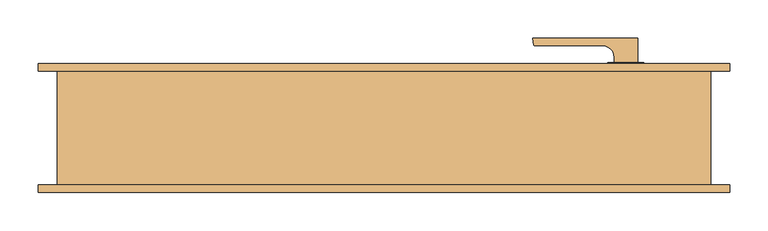
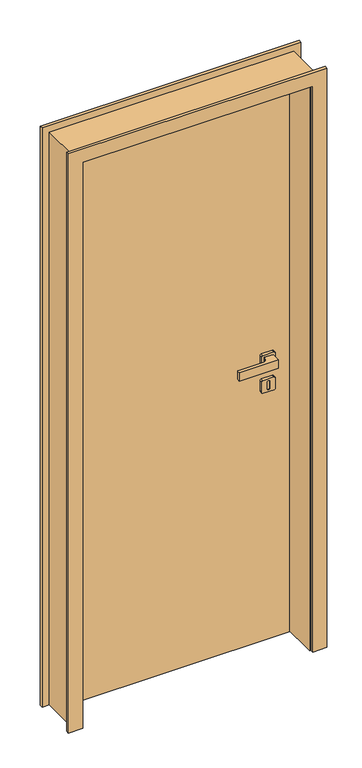
"""IFC4 building model written with IfcOpenShell, lengths in millimetres: door geometry, porta multiplas_growarq : porta giro simples 80 cm_growarq."""

import ifcopenshell
import ifcopenshell.guid

model = None  # the IFC model being written
_history = None  # IfcOwnerHistory: only IFC2X3 demands one
_inside = {}  # id of a spatial element -> (the spatial element, [elements in it])
_under = {}  # id of a project, library or spatial element -> (it, [spatial elements below it])
_declared = {}  # id of a project -> (the project, [libraries it declares])
_typed = {}  # id of a type object -> (the type object, [elements of that type])
_made_of = {}  # id of a material, layer set ... -> (it, [elements and type objects made of it])


def new_model(schema):
    """Start an empty IFC model of exactly this schema.

    Asked for "IFC4X3", IfcOpenShell would pick the latest addendum, in which some entities
    have other attributes; the version numbers below select the first issue.
    IFC2X3 requires an IfcOwnerHistory on every rooted entity: one is made here for all.
    """
    global model, _history
    if schema == "IFC4X3":
        model = ifcopenshell.file(schema_version=(4, 3, 0, 0))
    else:
        model = ifcopenshell.file(schema=schema)
    _inside.clear()
    _under.clear()
    _declared.clear()
    _typed.clear()
    _made_of.clear()
    _history = None
    if model.schema == "IFC2X3":
        org = make("IfcOrganization", Name="unknown")
        user = make(
            "IfcPersonAndOrganization",
            ThePerson=make("IfcPerson", FamilyName="unknown"),
            TheOrganization=org,
        )
        app = make(
            "IfcApplication",
            ApplicationDeveloper=org,
            Version="unknown",
            ApplicationFullName="unknown",
            ApplicationIdentifier="unknown",
        )
        _history = make(
            "IfcOwnerHistory",
            OwningUser=user,
            OwningApplication=app,
            ChangeAction="ADDED",
            CreationDate=0,
        )
    return model


def make(cls, **values):
    """One entity of the class cls with the attributes given. An attribute that is None is left unset."""
    return model.create_entity(
        cls, **{name: value for name, value in values.items() if value is not None}
    )


def rooted(cls, **values):
    """An entity with a GlobalId (a new one), such as an element, a storey or a relation."""
    return make(cls, GlobalId=ifcopenshell.guid.new(), OwnerHistory=_history, **values)


def si_unit(unit_type, name, prefix=None):
    """IfcSIUnit, for example si_unit("LENGTHUNIT", "METRE", prefix="MILLI")."""
    return make("IfcSIUnit", UnitType=unit_type, Prefix=prefix, Name=name)


def assignment(units):
    """IfcUnitAssignment: the units of a project."""
    return None if units is None else make("IfcUnitAssignment", Units=units)


def point(xyz):
    """IfcCartesianPoint."""
    return None if xyz is None else make("IfcCartesianPoint", Coordinates=xyz)


def direction(xyz):
    """IfcDirection."""
    return None if xyz is None else make("IfcDirection", DirectionRatios=xyz)


def frame(location, z_axis=None, x_axis=None):
    """IfcAxis2Placement3D, a coordinate frame: its origin and axes. An axis left out is left unset."""
    return make(
        "IfcAxis2Placement3D",
        Location=point(location),
        Axis=direction(z_axis),
        RefDirection=direction(x_axis),
    )


def frame_2d(location, x_axis=None):
    """IfcAxis2Placement2D, a coordinate frame in the plane: its origin and x axis."""
    return make(
        "IfcAxis2Placement2D", Location=point(location), RefDirection=direction(x_axis)
    )


def origin():
    """The frame at (0, 0, 0) with its axes left unset."""
    return frame((0.0, 0.0, 0.0))


def origin_with_axes():
    """The frame at (0, 0, 0) with the z axis (0, 0, 1) and the x axis (1, 0, 0) written out."""
    return frame((0.0, 0.0, 0.0), z_axis=(0.0, 0.0, 1.0), x_axis=(1.0, 0.0, 0.0))


def place(relative_to, where):
    """IfcLocalPlacement: puts the frame where relative to a parent placement (None: the world)."""
    return make(
        "IfcLocalPlacement", PlacementRelTo=relative_to, RelativePlacement=where
    )


def context(
    kind, dimensions, precision=None, world=None, true_north=None, identifier=None
):
    """IfcGeometricRepresentationContext, for example the 3D "Model" context."""
    return make(
        "IfcGeometricRepresentationContext",
        ContextIdentifier=identifier,
        ContextType=kind,
        CoordinateSpaceDimension=dimensions,
        Precision=precision,
        WorldCoordinateSystem=world,
        TrueNorth=true_north,
    )


def project(units=None, contexts=None):
    """IfcProject with its units and contexts."""
    return rooted(
        "IfcProject",
        Name="project",
        RepresentationContexts=contexts,
        UnitsInContext=assignment(units),
    )


def spatial(cls, under=None, at=None, **own):
    """A site, building, storey or space (cls), placed at a placement, below another one or the project."""
    s = rooted(cls, ObjectPlacement=at, **own)
    if under is not None:
        _under.setdefault(under.id(), (under, []))[1].append(s)
    return s


def polyline(points):
    """IfcPolyline through the points."""
    return make("IfcPolyline", Points=[point(p) for p in points])


def circle_curve(where, radius):
    """IfcCircle in the frame where."""
    return make("IfcCircle", Position=where, Radius=radius)


def trimmed(basis, trim1, trim2, sense, master):
    """IfcTrimmedCurve: the piece of a basis curve between two trims."""
    return make(
        "IfcTrimmedCurve",
        BasisCurve=basis,
        Trim1=trim1,
        Trim2=trim2,
        SenseAgreement=sense,
        MasterRepresentation=master,
    )


def segment(curve, same_sense, transition):
    """IfcCompositeCurveSegment."""
    return make(
        "IfcCompositeCurveSegment",
        Transition=transition,
        SameSense=same_sense,
        ParentCurve=curve,
    )


def composite_curve(segments, self_intersect=None):
    """IfcCompositeCurve: segments joined end to end."""
    return make("IfcCompositeCurve", Segments=segments, SelfIntersect=self_intersect)


def outline(outer, holes=None, kind="AREA"):
    """IfcArbitraryClosedProfileDef: a profile drawn as a closed curve; with holes, ...WithVoids."""
    if holes is None:
        return make("IfcArbitraryClosedProfileDef", ProfileType=kind, OuterCurve=outer)
    return make(
        "IfcArbitraryProfileDefWithVoids",
        ProfileType=kind,
        OuterCurve=outer,
        InnerCurves=holes,
    )


def extrude(swept, where, along, depth):
    """IfcExtrudedAreaSolid: the profile swept, set in the frame where, extruded along a direction by depth."""
    return make(
        "IfcExtrudedAreaSolid",
        SweptArea=swept,
        Position=where,
        ExtrudedDirection=direction(along),
        Depth=depth,
    )


def shape(context_of_items, identifier, shape_type, items):
    """IfcShapeRepresentation: the items that make up one representation, for example the "Body"."""
    return make(
        "IfcShapeRepresentation",
        ContextOfItems=context_of_items,
        RepresentationIdentifier=identifier,
        RepresentationType=shape_type,
        Items=items,
    )


def source(mapping_origin, context_of_items, identifier, shape_type, items):
    """IfcRepresentationMap: a shape defined once, which mapped items show again and again."""
    return make(
        "IfcRepresentationMap",
        MappingOrigin=mapping_origin,
        MappedRepresentation=shape(context_of_items, identifier, shape_type, items),
    )


def transform(
    local_origin,
    x_axis=None,
    y_axis=None,
    z_axis=None,
    scale=None,
    scale2=None,
    scale3=None,
    uniform=True,
):
    """IfcCartesianTransformationOperator3D, or its non-uniform kind. x_axis, y_axis, z_axis: its Axis1, 2, 3."""
    if uniform:
        return make(
            "IfcCartesianTransformationOperator3D",
            Axis1=direction(x_axis),
            Axis2=direction(y_axis),
            LocalOrigin=point(local_origin),
            Scale=scale,
            Axis3=direction(z_axis),
        )
    return make(
        "IfcCartesianTransformationOperator3DnonUniform",
        Axis1=direction(x_axis),
        Axis2=direction(y_axis),
        LocalOrigin=point(local_origin),
        Scale=scale,
        Axis3=direction(z_axis),
        Scale2=scale2,
        Scale3=scale3,
    )


def mapped(mapping_source, mapping_target):
    """IfcMappedItem: shows the shape of a source again, moved by a transform."""
    return make(
        "IfcMappedItem", MappingSource=mapping_source, MappingTarget=mapping_target
    )


def made_of(thing, what):
    """Note that an element or type object is made of a material, layer set ...; save() writes the relation."""
    if what is not None:
        _made_of.setdefault(what.id(), (what, []))[1].append(thing)
    return thing


def element(
    cls,
    number,
    at=None,
    inside=None,
    cuts=None,
    type_object=None,
    material=None,
    context=None,
    identifier="Body",
    shape_type=None,
    held_by="IfcProductDefinitionShape",
    body=None,
    shapes=None,
    **own,
):
    """One element of the class cls, such as IfcWall. Its Tag is "e" and its number.

    at: its placement. inside: the storey or other place that contains it. cuts: it is an
    opening in that element (IfcRelVoidsElement). A single representation is given by context,
    identifier, shape_type and body (its items); several are given by shapes. held_by: the class
    of the entity that holds the representations. save() writes the other relations.
    """
    e = rooted(cls, Tag="e%d" % number, ObjectPlacement=at, **own)
    if body is not None:
        shapes = [shape(context, identifier, shape_type, body)]
    if shapes is not None:
        e.Representation = make(held_by, Representations=shapes)
    if inside is not None:
        _inside.setdefault(inside.id(), (inside, []))[1].append(e)
    if cuts is not None:
        rooted(
            "IfcRelVoidsElement", RelatingBuildingElement=cuts, RelatedOpeningElement=e
        )
    if type_object is not None:
        _typed.setdefault(type_object.id(), (type_object, []))[1].append(e)
    return made_of(e, material)


def aggregate(whole, parts):
    """IfcRelAggregates: a whole, such as a stair, and the parts it consists of."""
    return rooted("IfcRelAggregates", RelatingObject=whole, RelatedObjects=parts)


def save(model, path):
    """Write the relations noted so far, then the file.

    IfcRelAggregates (storeys below a building ...), IfcRelContainedInSpatialStructure (elements
    in a storey), IfcRelDefinesByType, IfcRelAssociatesMaterial and IfcRelDeclares: one each for
    every whole, place, type object, material and project.
    """
    for whole, parts in _under.values():
        aggregate(whole, parts)
    for where, things in _inside.values():
        rooted(
            "IfcRelContainedInSpatialStructure",
            RelatedElements=things,
            RelatingStructure=where,
        )
    for kind, things in _typed.values():
        rooted("IfcRelDefinesByType", RelatedObjects=things, RelatingType=kind)
    for what, things in _made_of.values():
        rooted("IfcRelAssociatesMaterial", RelatedObjects=things, RelatingMaterial=what)
    for by, libraries in _declared.values():
        rooted("IfcRelDeclares", RelatingContext=by, RelatedDefinitions=libraries)
    model.write(path)


def plane_surface(at):
    """IfcPlane: the flat surface through the origin of the frame at, square to its z axis."""
    return make("IfcPlane", Position=at)


def cylinder_surface(at, radius):
    """IfcCylindricalSurface: all points at the distance radius from the z axis of the frame at."""
    return make("IfcCylindricalSurface", Position=at, Radius=radius)


def revolved_surface(curve, axis_point, axis_direction):
    """IfcSurfaceOfRevolution: the curve turned about the line through axis_point along axis_direction."""
    return make(
        "IfcSurfaceOfRevolution",
        SweptCurve=make("IfcArbitraryOpenProfileDef", ProfileType="CURVE", Curve=curve),
        AxisPosition=make("IfcAxis1Placement", Location=point(axis_point), Axis=direction(axis_direction)),
    )


def advanced_brep(points, edges, surfaces, faces):
    """IfcAdvancedBrep: a solid bounded by faces that lie on surfaces and meet in shared edges.

    An edge is (start, end): straight between two places in points (the first is 0);
    or (start, end, curve); or (start, end, curve, False) where it runs against its curve.
    A face is (place in surfaces, loops), or (place, loops, False) where it looks against
    its surface's normal. A loop lists edges by number (the first is 1), with a minus sign
    where the edge is run from its end to its start. The first loop is the outer one.
    """
    corners = [point(p) for p in points]
    vertices = [make("IfcVertexPoint", VertexGeometry=c) for c in corners]
    made = []
    for start, end, *more in edges:
        made.append(
            make(
                "IfcEdgeCurve",
                EdgeStart=vertices[start],
                EdgeEnd=vertices[end],
                EdgeGeometry=more[0] if more else make("IfcPolyline", Points=[corners[start], corners[end]]),
                SameSense=more[1] if len(more) > 1 else True,
            )
        )
    hull = []
    for where, loops, *sense in faces:
        bounds = []
        for j, loop in enumerate(loops):
            ring = [make("IfcOrientedEdge", EdgeElement=made[abs(k) - 1], Orientation=k > 0) for k in loop]
            bounds.append(
                make(
                    "IfcFaceOuterBound" if j == 0 else "IfcFaceBound",
                    Bound=make("IfcEdgeLoop", EdgeList=ring),
                    Orientation=True,
                )
            )
        hull.append(make("IfcAdvancedFace", Bounds=bounds, FaceSurface=surfaces[where], SameSense=sense[0] if sense else True))
    return make("IfcAdvancedBrep", Outer=make("IfcClosedShell", CfsFaces=hull))


def door_262d71ed(model_context):
    return source(origin(), model_context, "Body", "SolidModel", [
        advanced_brep(
        [(337.5247906, 86.0, 975.2140175), (341.5247906, 86.0, 971.2140175), (341.5247906, 86.0, 932.3348635), (337.5247906, 86.0, 928.3348635), (298.475196, 86.0, 928.3348635), (294.475196, 86.0, 932.3348635), (294.475196, 86.0, 971.2071442), (298.4820692, 86.0, 975.2140175), (323.0036235, 86.0, 963.1453546), (312.9935514, 86.0, 963.1453546), (312.9935514, 86.0, 940.4035264), (323.0036235, 86.0, 940.4035264), (337.5247906, 75.0, 975.2140175), (298.4820692, 75.0, 975.2140175), (294.475196, 75.0, 971.2071442), (294.475196, 75.0, 932.3348635), (298.475196, 75.0, 928.3348635), (337.5247906, 75.0, 928.3348635), (341.5247906, 75.0, 932.3348635), (341.5247906, 75.0, 971.2140175), (323.0036235, 84.0, 940.4035264), (312.9935514, 84.0, 940.4035264), (312.9935514, 84.0, 963.1453546), (323.0036235, 84.0, 963.1453546)],
        [
            (0, 1, circle_curve(frame((337.5247906, 86.0, 971.2140175), z_axis=(0.0, 1.0, 0.0), x_axis=(1.0, 0.0, 0.0)), 4.0)),
            (1, 2),
            (2, 3, circle_curve(frame((337.5247906, 86.0, 932.3348635), z_axis=(0.0, 1.0, 0.0), x_axis=(1.0, 0.0, 0.0)), 4.0)),
            (3, 4),
            (4, 5, circle_curve(frame((298.475196, 86.0, 932.3348635), z_axis=(0.0, 1.0, 0.0), x_axis=(1.0, 0.0, 0.0)), 4.0)),
            (5, 6),
            (6, 7, circle_curve(frame((298.4820692, 86.0, 971.2071442), z_axis=(0.0, 1.0, 0.0), x_axis=(1.0, 0.0, 0.0)), 4.0068732)),
            (7, 0),
            (8, 9, circle_curve(frame((317.9985874, 86.0, 963.1453546), z_axis=(0.0, -1.0, 0.0), x_axis=(1.0, 0.0, 0.0)), 5.0050361)),
            (9, 10),
            (10, 11, circle_curve(frame((317.9985874, 86.0, 940.4035264), z_axis=(0.0, -1.0, 0.0), x_axis=(1.0, 0.0, 0.0)), 5.0050361)),
            (11, 8),
            (12, 13),
            (13, 14, circle_curve(frame((298.4820692, 75.0, 971.2071442), z_axis=(0.0, -1.0, 0.0), x_axis=(1.0, 0.0, 0.0)), 4.0068732)),
            (14, 15),
            (15, 16, circle_curve(frame((298.475196, 75.0, 932.3348635), z_axis=(0.0, -1.0, 0.0), x_axis=(1.0, 0.0, 0.0)), 4.0)),
            (16, 17),
            (17, 18, circle_curve(frame((337.5247906, 75.0, 932.3348635), z_axis=(0.0, -1.0, 0.0), x_axis=(1.0, 0.0, 0.0)), 4.0)),
            (18, 19),
            (19, 12, circle_curve(frame((337.5247906, 75.0, 971.2140175), z_axis=(0.0, -1.0, 0.0), x_axis=(1.0, 0.0, 0.0)), 4.0)),
            (7, 13),
            (12, 0),
            (6, 14),
            (5, 15),
            (4, 16),
            (3, 17),
            (2, 18),
            (1, 19),
            (20, 21, circle_curve(frame((317.9985874, 84.0, 940.4035264), z_axis=(0.0, 1.0, 0.0), x_axis=(1.0, 0.0, 0.0)), 5.0050361)),
            (21, 22),
            (22, 23, circle_curve(frame((317.9985874, 84.0, 963.1453546), z_axis=(0.0, 1.0, 0.0), x_axis=(1.0, 0.0, 0.0)), 5.0050361)),
            (23, 20),
            (23, 8),
            (11, 20),
            (21, 10),
            (9, 22),
        ],
        [
            plane_surface(frame((298.4781039, 86.0, 975.2140175), z_axis=(0.0, 1.0, 0.0), x_axis=(-1.0, 0.0, 0.0))),
            plane_surface(frame((298.4781039, 75.0, 975.2140175), z_axis=(0.0, -1.0, 0.0), x_axis=(1.0, 0.0, 0.0))),
            plane_surface(frame((337.5247906, 86.0, 975.2140175), z_axis=(0.0, 0.0, 1.0), x_axis=(0.0, -1.0, 0.0))),
            cylinder_surface(frame((298.4820692, 75.0, 971.2071442), z_axis=(0.0, 1.0, 0.0), x_axis=(1.0, 0.0, 0.0)), 4.0068732),
            plane_surface(frame((294.475196, 86.0, 971.2071442), z_axis=(-1.0, 0.0, 0.0), x_axis=(0.0, -1.0, 0.0))),
            cylinder_surface(frame((298.475196, 75.0, 932.3348635), z_axis=(0.0, 1.0, 0.0), x_axis=(1.0, 0.0, 0.0)), 4.0),
            plane_surface(frame((298.475196, 86.0, 928.3348635), z_axis=(0.0, 0.0, -1.0), x_axis=(0.0, -1.0, 0.0))),
            cylinder_surface(frame((337.5247906, 75.0, 932.3348635), z_axis=(0.0, 1.0, 0.0), x_axis=(1.0, 0.0, 0.0)), 4.0),
            plane_surface(frame((341.5247906, 86.0, 932.3348635), z_axis=(1.0, 0.0, 0.0), x_axis=(0.0, -1.0, 0.0))),
            cylinder_surface(frame((337.5247906, 75.0, 971.2140175), z_axis=(0.0, 1.0, 0.0), x_axis=(1.0, 0.0, 0.0)), 4.0),
            plane_surface(frame((323.0036235, 84.0, 952.9958878), z_axis=(0.0, 1.0, 0.0), x_axis=(0.0, 0.0, -1.0))),
            plane_surface(frame((323.0036235, 86.0, 940.4035264), z_axis=(-1.0, 0.0, 0.0), x_axis=(0.0, -1.0, 0.0))),
            plane_surface(frame((312.9935514, 86.0, 963.1453546), z_axis=(1.0, 0.0, 0.0), x_axis=(0.0, -1.0, 0.0))),
            revolved_surface(polyline([(323.0036235, 86.0, 940.4035264), (323.0036235, 84.0, 940.4035264)]), (317.9985874, 84.0, 940.4035264), (0.0, 1.0, 0.0)),
            revolved_surface(polyline([(323.0036235, 86.0, 963.1453546), (323.0036235, 84.0, 963.1453546)]), (317.9985874, 84.0, 963.1453546), (0.0, 1.0, 0.0)),
        ],
        [
            (0, [[1, 2, 3, 4, 5, 6, 7, 8], [9, 10, 11, 12]]),
            (1, [[13, 14, 15, 16, 17, 18, 19, 20]]),
            (2, [[21, -13, 22, -8]]),
            (3, [[23, -14, -21, -7]]),
            (4, [[24, -15, -23, -6]]),
            (5, [[25, -16, -24, -5]]),
            (6, [[26, -17, -25, -4]]),
            (7, [[27, -18, -26, -3]]),
            (8, [[28, -19, -27, -2]]),
            (9, [[-22, -20, -28, -1]]),
            (10, [[29, 30, 31, 32]]),
            (11, [[33, -12, 34, -32]]),
            (12, [[35, -10, 36, -30]]),
            (13, [[-34, -11, -35, -29]]),
            (14, [[-36, -9, -33, -31]]),
        ],
    ),
        advanced_brep(
        [(337.5247906, 86.0, 1068.227973), (341.5247906, 86.0, 1064.227973), (341.5247906, 86.0, 1025.3488191), (337.5247906, 86.0, 1021.3488191), (298.475196, 86.0, 1021.3488191), (294.475196, 86.0, 1025.3488191), (294.475196, 86.0, 1064.2210998), (298.4820692, 86.0, 1068.227973), (337.5247906, 75.0, 1068.227973), (298.4820692, 75.0, 1068.227973), (294.475196, 75.0, 1064.2210998), (294.475196, 75.0, 1025.3488191), (298.475196, 75.0, 1021.3488191), (337.5247906, 75.0, 1021.3488191), (341.5247906, 75.0, 1025.3488191), (341.5247906, 75.0, 1064.227973)],
        [
            (0, 1, circle_curve(frame((337.5247906, 86.0, 1064.227973), z_axis=(0.0, 1.0, 0.0), x_axis=(1.0, 0.0, 0.0)), 4.0)),
            (1, 2),
            (2, 3, circle_curve(frame((337.5247906, 86.0, 1025.3488191), z_axis=(0.0, 1.0, 0.0), x_axis=(1.0, 0.0, 0.0)), 4.0)),
            (3, 4),
            (4, 5, circle_curve(frame((298.475196, 86.0, 1025.3488191), z_axis=(0.0, 1.0, 0.0), x_axis=(1.0, 0.0, 0.0)), 4.0)),
            (5, 6),
            (6, 7, circle_curve(frame((298.4820692, 86.0, 1064.2210998), z_axis=(0.0, 1.0, 0.0), x_axis=(1.0, 0.0, 0.0)), 4.0068732)),
            (7, 0),
            (8, 9),
            (9, 10, circle_curve(frame((298.4820692, 75.0, 1064.2210998), z_axis=(0.0, -1.0, 0.0), x_axis=(1.0, 0.0, 0.0)), 4.0068732)),
            (10, 11),
            (11, 12, circle_curve(frame((298.475196, 75.0, 1025.3488191), z_axis=(0.0, -1.0, 0.0), x_axis=(1.0, 0.0, 0.0)), 4.0)),
            (12, 13),
            (13, 14, circle_curve(frame((337.5247906, 75.0, 1025.3488191), z_axis=(0.0, -1.0, 0.0), x_axis=(1.0, 0.0, 0.0)), 4.0)),
            (14, 15),
            (15, 8, circle_curve(frame((337.5247906, 75.0, 1064.227973), z_axis=(0.0, -1.0, 0.0), x_axis=(1.0, 0.0, 0.0)), 4.0)),
            (7, 9),
            (8, 0),
            (6, 10),
            (5, 11),
            (4, 12),
            (3, 13),
            (2, 14),
            (1, 15),
        ],
        [
            plane_surface(frame((298.4781039, 86.0, 975.2140175), z_axis=(0.0, 1.0, 0.0), x_axis=(-1.0, 0.0, 0.0))),
            plane_surface(frame((298.4781039, 75.0, 975.2140175), z_axis=(0.0, -1.0, 0.0), x_axis=(1.0, 0.0, 0.0))),
            plane_surface(frame((337.5247906, 86.0, 1068.227973), z_axis=(0.0, 0.0, 1.0), x_axis=(0.0, -1.0, 0.0))),
            cylinder_surface(frame((298.4820692, 75.0, 1064.2210998), z_axis=(0.0, 1.0, 0.0), x_axis=(1.0, 0.0, 0.0)), 4.0068732),
            plane_surface(frame((294.475196, 86.0, 1064.2210998), z_axis=(-1.0, 0.0, 0.0), x_axis=(0.0, -1.0, 0.0))),
            cylinder_surface(frame((298.475196, 75.0, 1025.3488191), z_axis=(0.0, 1.0, 0.0), x_axis=(1.0, 0.0, 0.0)), 4.0),
            plane_surface(frame((298.475196, 86.0, 1021.3488191), z_axis=(0.0, 0.0, -1.0), x_axis=(0.0, -1.0, 0.0))),
            cylinder_surface(frame((337.5247906, 75.0, 1025.3488191), z_axis=(0.0, 1.0, 0.0), x_axis=(1.0, 0.0, 0.0)), 4.0),
            plane_surface(frame((341.5247906, 86.0, 1025.3488191), z_axis=(1.0, 0.0, 0.0), x_axis=(0.0, -1.0, 0.0))),
            cylinder_surface(frame((337.5247906, 75.0, 1064.227973), z_axis=(0.0, 1.0, 0.0), x_axis=(1.0, 0.0, 0.0)), 4.0),
        ],
        [
            (0, [[1, 2, 3, 4, 5, 6, 7, 8]]),
            (1, [[9, 10, 11, 12, 13, 14, 15, 16]]),
            (2, [[17, -9, 18, -8]]),
            (3, [[19, -10, -17, -7]]),
            (4, [[20, -11, -19, -6]]),
            (5, [[21, -12, -20, -5]]),
            (6, [[22, -13, -21, -4]]),
            (7, [[23, -14, -22, -3]]),
            (8, [[24, -15, -23, -2]]),
            (9, [[-18, -16, -24, -1]]),
        ],
    ),
        extrude(outline(composite_curve([segment(polyline([(333.5247906, 118.5150355), (333.5247906, 86.7793682), (302.475196, 86.7793682), (302.475196, 93.5981558)]), True, "CONTINUOUS"), segment(trimmed(circle_curve(frame_2d((287.4483579, 93.5981558)), 15.0268381), [point((302.475196, 93.5981558))], [point((287.4483579, 108.6249939))], True, "CARTESIAN"), True, "CONTINUOUS"), segment(polyline([(287.4483579, 108.6249939), (198.1590205, 108.6249939)]), True, "CONTINUOUS"), segment(trimmed(circle_curve(frame_2d((198.1590205, 109.6372538)), 1.0122598), [point((198.1590205, 108.6249939))], [point((197.1621392, 109.4614767))], False, "CARTESIAN"), True, "CONTINUOUS"), segment(polyline([(197.1621392, 109.4614767), (195.5657525, 118.5150355), (333.5247906, 118.5150355)]), True, "CONTINUOUS")], self_intersect=False)), frame((0.0, 0.0, 1029.3488191), z_axis=(0.0, 0.0, 1.0), x_axis=(1.0, 0.0, 0.0)), (0.0, 0.0, 1.0), 30.8791539),
        advanced_brep(
        [(337.5247906, 34.0, 975.2140175), (298.4820692, 34.0, 975.2140175), (294.475196, 34.0, 971.2071442), (294.475196, 34.0, 932.3348635), (298.475196, 34.0, 928.3348635), (337.5247906, 34.0, 928.3348635), (341.5247906, 34.0, 932.3348635), (341.5247906, 34.0, 971.2140175), (323.0036235, 34.0, 963.1453546), (323.0036235, 34.0, 940.4035264), (312.9935514, 34.0, 940.4035264), (312.9935514, 34.0, 963.1453546), (337.5247906, 45.0, 975.2140175), (341.5247906, 45.0, 971.2140175), (341.5247906, 45.0, 932.3348635), (337.5247906, 45.0, 928.3348635), (298.475196, 45.0, 928.3348635), (294.475196, 45.0, 932.3348635), (294.475196, 45.0, 971.2071442), (298.4820692, 45.0, 975.2140175), (323.0036235, 36.0, 940.4035264), (323.0036235, 36.0, 963.1453546), (312.9935514, 36.0, 963.1453546), (312.9935514, 36.0, 940.4035264)],
        [
            (0, 1),
            (1, 2, circle_curve(frame((298.4820692, 34.0, 971.2071442), z_axis=(0.0, -1.0, 0.0), x_axis=(1.0, 0.0, 0.0)), 4.0068732)),
            (2, 3),
            (3, 4, circle_curve(frame((298.475196, 34.0, 932.3348635), z_axis=(0.0, -1.0, 0.0), x_axis=(1.0, 0.0, 0.0)), 4.0)),
            (4, 5),
            (5, 6, circle_curve(frame((337.5247906, 34.0, 932.3348635), z_axis=(0.0, -1.0, 0.0), x_axis=(1.0, 0.0, 0.0)), 4.0)),
            (6, 7),
            (7, 0, circle_curve(frame((337.5247906, 34.0, 971.2140175), z_axis=(0.0, -1.0, 0.0), x_axis=(1.0, 0.0, 0.0)), 4.0)),
            (8, 9),
            (9, 10, circle_curve(frame((317.9985874, 34.0, 940.4035264), z_axis=(0.0, 1.0, 0.0), x_axis=(1.0, 0.0, 0.0)), 5.0050361)),
            (10, 11),
            (11, 8, circle_curve(frame((317.9985874, 34.0, 963.1453546), z_axis=(0.0, 1.0, 0.0), x_axis=(1.0, 0.0, 0.0)), 5.0050361)),
            (12, 13, circle_curve(frame((337.5247906, 45.0, 971.2140175), z_axis=(0.0, 1.0, 0.0), x_axis=(1.0, 0.0, 0.0)), 4.0)),
            (13, 14),
            (14, 15, circle_curve(frame((337.5247906, 45.0, 932.3348635), z_axis=(0.0, 1.0, 0.0), x_axis=(1.0, 0.0, 0.0)), 4.0)),
            (15, 16),
            (16, 17, circle_curve(frame((298.475196, 45.0, 932.3348635), z_axis=(0.0, 1.0, 0.0), x_axis=(1.0, 0.0, 0.0)), 4.0)),
            (17, 18),
            (18, 19, circle_curve(frame((298.4820692, 45.0, 971.2071442), z_axis=(0.0, 1.0, 0.0), x_axis=(1.0, 0.0, 0.0)), 4.0068732)),
            (19, 12),
            (0, 12),
            (19, 1),
            (18, 2),
            (17, 3),
            (16, 4),
            (15, 5),
            (14, 6),
            (13, 7),
            (20, 21),
            (21, 22, circle_curve(frame((317.9985874, 36.0, 963.1453546), z_axis=(0.0, -1.0, 0.0), x_axis=(1.0, 0.0, 0.0)), 5.0050361)),
            (22, 23),
            (23, 20, circle_curve(frame((317.9985874, 36.0, 940.4035264), z_axis=(0.0, -1.0, 0.0), x_axis=(1.0, 0.0, 0.0)), 5.0050361)),
            (20, 9),
            (8, 21),
            (22, 11),
            (10, 23),
        ],
        [
            plane_surface(frame((298.4781039, 34.0, 975.2140175), z_axis=(0.0, -1.0, 0.0), x_axis=(-1.0, 0.0, 0.0))),
            plane_surface(frame((298.4781039, 45.0, 975.2140175), z_axis=(0.0, 1.0, 0.0), x_axis=(1.0, 0.0, 0.0))),
            plane_surface(frame((337.5247906, 34.0, 975.2140175), z_axis=(0.0, 0.0, 1.0), x_axis=(0.0, 1.0, 0.0))),
            cylinder_surface(frame((298.4820692, 45.0, 971.2071442), z_axis=(0.0, -1.0, 0.0), x_axis=(1.0, 0.0, 0.0)), 4.0068732),
            plane_surface(frame((294.475196, 34.0, 971.2071442), z_axis=(-1.0, 0.0, 0.0), x_axis=(0.0, 1.0, 0.0))),
            cylinder_surface(frame((298.475196, 45.0, 932.3348635), z_axis=(0.0, -1.0, 0.0), x_axis=(1.0, 0.0, 0.0)), 4.0),
            plane_surface(frame((298.475196, 34.0, 928.3348635), z_axis=(0.0, 0.0, -1.0), x_axis=(0.0, 1.0, 0.0))),
            cylinder_surface(frame((337.5247906, 45.0, 932.3348635), z_axis=(0.0, -1.0, 0.0), x_axis=(1.0, 0.0, 0.0)), 4.0),
            plane_surface(frame((341.5247906, 34.0, 932.3348635), z_axis=(1.0, 0.0, 0.0), x_axis=(0.0, 1.0, 0.0))),
            cylinder_surface(frame((337.5247906, 45.0, 971.2140175), z_axis=(0.0, -1.0, 0.0), x_axis=(1.0, 0.0, 0.0)), 4.0),
            plane_surface(frame((323.0036235, 36.0, 952.9958878), z_axis=(0.0, -1.0, 0.0), x_axis=(0.0, 0.0, -1.0))),
            plane_surface(frame((323.0036235, 34.0, 940.4035264), z_axis=(-1.0, 0.0, 0.0), x_axis=(0.0, 1.0, 0.0))),
            plane_surface(frame((312.9935514, 34.0, 963.1453546), z_axis=(1.0, 0.0, 0.0), x_axis=(0.0, 1.0, 0.0))),
            revolved_surface(polyline([(323.0036235, 34.0, 940.4035264), (323.0036235, 36.0, 940.4035264)]), (317.9985874, 36.0, 940.4035264), (0.0, -1.0, 0.0)),
            revolved_surface(polyline([(323.0036235, 34.0, 963.1453546), (323.0036235, 36.0, 963.1453546)]), (317.9985874, 36.0, 963.1453546), (0.0, -1.0, 0.0)),
        ],
        [
            (0, [[1, 2, 3, 4, 5, 6, 7, 8], [9, 10, 11, 12]]),
            (1, [[13, 14, 15, 16, 17, 18, 19, 20]]),
            (2, [[-1, 21, -20, 22]]),
            (3, [[-2, -22, -19, 23]]),
            (4, [[-3, -23, -18, 24]]),
            (5, [[-4, -24, -17, 25]]),
            (6, [[-5, -25, -16, 26]]),
            (7, [[-6, -26, -15, 27]]),
            (8, [[-7, -27, -14, 28]]),
            (9, [[-8, -28, -13, -21]]),
            (10, [[29, 30, 31, 32]]),
            (11, [[-29, 33, -9, 34]]),
            (12, [[-31, 35, -11, 36]]),
            (13, [[-32, -36, -10, -33]]),
            (14, [[-30, -34, -12, -35]]),
        ],
    ),
        advanced_brep(
        [(337.5247906, 34.0, 1068.227973), (298.4820692, 34.0, 1068.227973), (294.475196, 34.0, 1064.2210998), (294.475196, 34.0, 1025.3488191), (298.475196, 34.0, 1021.3488191), (337.5247906, 34.0, 1021.3488191), (341.5247906, 34.0, 1025.3488191), (341.5247906, 34.0, 1064.227973), (337.5247906, 45.0, 1068.227973), (341.5247906, 45.0, 1064.227973), (341.5247906, 45.0, 1025.3488191), (337.5247906, 45.0, 1021.3488191), (298.475196, 45.0, 1021.3488191), (294.475196, 45.0, 1025.3488191), (294.475196, 45.0, 1064.2210998), (298.4820692, 45.0, 1068.227973)],
        [
            (0, 1),
            (1, 2, circle_curve(frame((298.4820692, 34.0, 1064.2210998), z_axis=(0.0, -1.0, 0.0), x_axis=(1.0, 0.0, 0.0)), 4.0068732)),
            (2, 3),
            (3, 4, circle_curve(frame((298.475196, 34.0, 1025.3488191), z_axis=(0.0, -1.0, 0.0), x_axis=(1.0, 0.0, 0.0)), 4.0)),
            (4, 5),
            (5, 6, circle_curve(frame((337.5247906, 34.0, 1025.3488191), z_axis=(0.0, -1.0, 0.0), x_axis=(1.0, 0.0, 0.0)), 4.0)),
            (6, 7),
            (7, 0, circle_curve(frame((337.5247906, 34.0, 1064.227973), z_axis=(0.0, -1.0, 0.0), x_axis=(1.0, 0.0, 0.0)), 4.0)),
            (8, 9, circle_curve(frame((337.5247906, 45.0, 1064.227973), z_axis=(0.0, 1.0, 0.0), x_axis=(1.0, 0.0, 0.0)), 4.0)),
            (9, 10),
            (10, 11, circle_curve(frame((337.5247906, 45.0, 1025.3488191), z_axis=(0.0, 1.0, 0.0), x_axis=(1.0, 0.0, 0.0)), 4.0)),
            (11, 12),
            (12, 13, circle_curve(frame((298.475196, 45.0, 1025.3488191), z_axis=(0.0, 1.0, 0.0), x_axis=(1.0, 0.0, 0.0)), 4.0)),
            (13, 14),
            (14, 15, circle_curve(frame((298.4820692, 45.0, 1064.2210998), z_axis=(0.0, 1.0, 0.0), x_axis=(1.0, 0.0, 0.0)), 4.0068732)),
            (15, 8),
            (0, 8),
            (15, 1),
            (14, 2),
            (13, 3),
            (12, 4),
            (11, 5),
            (10, 6),
            (9, 7),
        ],
        [
            plane_surface(frame((298.4781039, 34.0, 975.2140175), z_axis=(0.0, -1.0, 0.0), x_axis=(-1.0, 0.0, 0.0))),
            plane_surface(frame((298.4781039, 45.0, 975.2140175), z_axis=(0.0, 1.0, 0.0), x_axis=(1.0, 0.0, 0.0))),
            plane_surface(frame((337.5247906, 34.0, 1068.227973), z_axis=(0.0, 0.0, 1.0), x_axis=(0.0, 1.0, 0.0))),
            cylinder_surface(frame((298.4820692, 45.0, 1064.2210998), z_axis=(0.0, -1.0, 0.0), x_axis=(1.0, 0.0, 0.0)), 4.0068732),
            plane_surface(frame((294.475196, 34.0, 1064.2210998), z_axis=(-1.0, 0.0, 0.0), x_axis=(0.0, 1.0, 0.0))),
            cylinder_surface(frame((298.475196, 45.0, 1025.3488191), z_axis=(0.0, -1.0, 0.0), x_axis=(1.0, 0.0, 0.0)), 4.0),
            plane_surface(frame((298.475196, 34.0, 1021.3488191), z_axis=(0.0, 0.0, -1.0), x_axis=(0.0, 1.0, 0.0))),
            cylinder_surface(frame((337.5247906, 45.0, 1025.3488191), z_axis=(0.0, -1.0, 0.0), x_axis=(1.0, 0.0, 0.0)), 4.0),
            plane_surface(frame((341.5247906, 34.0, 1025.3488191), z_axis=(1.0, 0.0, 0.0), x_axis=(0.0, 1.0, 0.0))),
            cylinder_surface(frame((337.5247906, 45.0, 1064.227973), z_axis=(0.0, -1.0, 0.0), x_axis=(1.0, 0.0, 0.0)), 4.0),
        ],
        [
            (0, [[1, 2, 3, 4, 5, 6, 7, 8]]),
            (1, [[9, 10, 11, 12, 13, 14, 15, 16]]),
            (2, [[-1, 17, -16, 18]]),
            (3, [[-2, -18, -15, 19]]),
            (4, [[-3, -19, -14, 20]]),
            (5, [[-4, -20, -13, 21]]),
            (6, [[-5, -21, -12, 22]]),
            (7, [[-6, -22, -11, 23]]),
            (8, [[-7, -23, -10, 24]]),
            (9, [[-8, -24, -9, -17]]),
        ],
    ),
        extrude(outline(composite_curve([segment(polyline([(333.5247906, 1.4849645), (195.5657525, 1.4849645), (197.1621392, 10.5385233)]), True, "CONTINUOUS"), segment(trimmed(circle_curve(frame_2d((198.1590205, 10.3627462)), 1.0122598), [point((197.1621392, 10.5385233))], [point((198.1590205, 11.3750061))], False, "CARTESIAN"), True, "CONTINUOUS"), segment(polyline([(198.1590205, 11.3750061), (287.4483579, 11.3750061)]), True, "CONTINUOUS"), segment(trimmed(circle_curve(frame_2d((287.4483579, 26.4018442)), 15.0268381), [point((287.4483579, 11.3750061))], [point((302.475196, 26.4018442))], True, "CARTESIAN"), True, "CONTINUOUS"), segment(polyline([(302.475196, 26.4018442), (302.475196, 33.2206318), (333.5247906, 33.2206318), (333.5247906, 1.4849645)]), True, "CONTINUOUS")], self_intersect=False)), frame((0.0, 0.0, 1029.3488191), z_axis=(0.0, 0.0, 1.0), x_axis=(1.0, 0.0, 0.0)), (0.0, 0.0, 1.0), 30.8791539),
        extrude(outline(polyline([(398.0, 45.0), (-398.0, 45.0), (-398.0, 75.0), (398.0, 75.0), (398.0, 45.0)])), origin_with_axes(), (0.0, 0.0, 1.0), 2098.0),
        extrude(outline(polyline([(0.0, 400.0), (0.0, 430.0), (2130.0, 430.0), (2130.0, -430.0), (0.0, -430.0), (0.0, -400.0), (2100.0, -400.0), (2100.0, 400.0), (0.0, 400.0)])), frame((0.0, -75.0, 0.0), z_axis=(0.0, 1.0, 0.0), x_axis=(0.0, 0.0, 1.0)), (0.0, 0.0, 1.0), 150.0),
        extrude(outline(polyline([(2155.0, -455.0), (0.0, -455.0), (0.0, -405.0), (2105.0, -405.0), (2105.0, 405.0), (0.0, 405.0), (0.0, 455.0), (2155.0, 455.0), (2155.0, -455.0)])), frame((0.0, -85.0, 0.0), z_axis=(0.0, 1.0, 0.0), x_axis=(0.0, 0.0, 1.0)), (0.0, 0.0, 1.0), 10.0),
        extrude(outline(polyline([(2105.0, 405.0), (0.0, 405.0), (0.0, 455.0), (2155.0, 455.0), (2155.0, -455.0), (0.0, -455.0), (0.0, -405.0), (2105.0, -405.0), (2105.0, 405.0)])), frame((0.0, 75.0, 0.0), z_axis=(0.0, 1.0, 0.0), x_axis=(0.0, 0.0, 1.0)), (0.0, 0.0, 1.0), 10.0),
    ])


if __name__ == "__main__":
    model = new_model("IFC4")
    model_context = context("Model", 3, world=origin())
    ifc_project = project(units=[si_unit("LENGTHUNIT", "METRE", prefix="MILLI")], contexts=[model_context])
    site = spatial("IfcSite", under=ifc_project)
    building = spatial("IfcBuilding", under=site)
    placement = place(None, origin())
    door_shape = door_262d71ed(model_context)
    element("IfcDoor", 1, ObjectType="porta multiplas_growarq : porta giro simples 80 cm_growarq", at=placement, inside=building, context=model_context, shape_type="MappedRepresentation", body=[
        mapped(door_shape, transform((0.0, 0.0, 0.0), x_axis=(1.0, 0.0, 0.0), y_axis=(0.0, 1.0, 0.0), z_axis=(0.0, 0.0, 1.0))),
    ])
    save(model, "model.ifc")

# Revit data of these elements
# Type "porta multiplas_growarq : porta giro simples 80 cm_growarq"
#   Type Mark = "P02"
#   Description = "Porta de Madeira com uma folha de abrir"
#   Analytic Construction = "<None>"
#   Cost = 0
#   Rough Width = 860 mm
#   Largura Guarnição = 50 mm
#   Espessura Guarnição = 10 mm
#   Thickness = 30 mm
#   Rough Height = 2130 mm
#   Marco = 30 mm
#   Largura Folha Eixo = 596 mm
#   Height = 2100 mm
#   Width = 800 mm
#   Largura Folha = 796 mm
#   Eixo = 200 mm
#   Altura Folha = 2098 mm
#   Abertura correr [instance default] = 200 mm
#   Abertura [instance default] = 0.00°
#   Simples = yes
#   Guarnição = yes
#   Eixo Folha = no
#   Dupla = no
#   Correr = no
#   Material = .pintura branca_growarq
#   Function = (empty or 0)
#   Wall Closure = (empty or 0)
# Element 1 (IfcDoor, "porta multiplas_growarq : porta giro simples 80 cm_growarq")
#   Materials on its faces: ".pintura branca_growarq"
# Materials
#   ".pintura branca_growarq": class "Pintura", colour RGB 255 255 255, transparency 0, Keynote = "0102", Comments = "Pintura com tinta látex na cor branca", Description = "Pintura branca", Cost = 0
